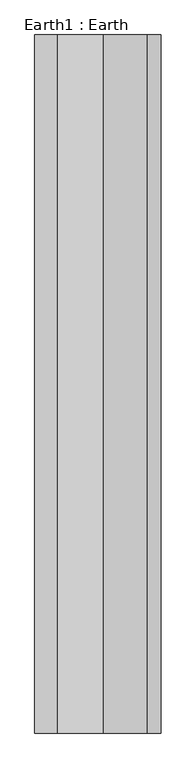
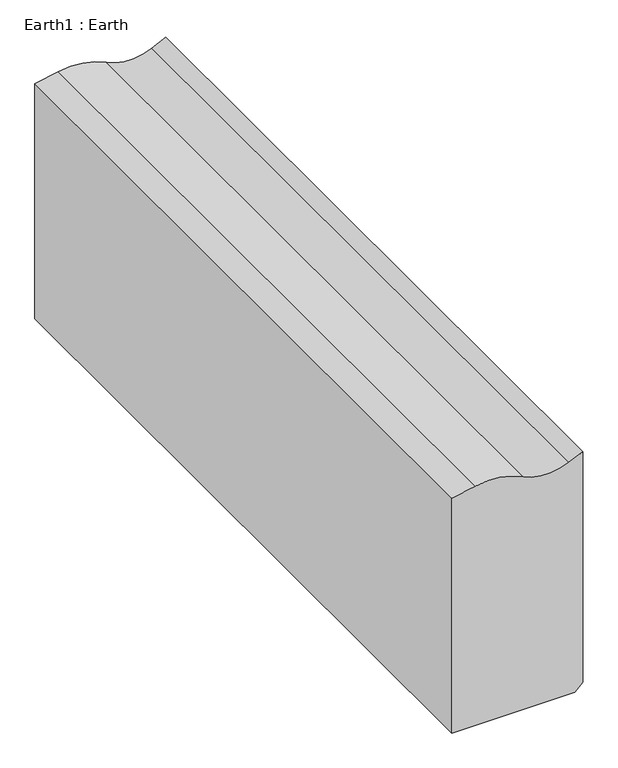
"""IFC4 building model written with IfcOpenShell, lengths in millimetres: proxy geometry, Earth1 : Earth."""

from ifc_helpers import new_model, si_unit, point, frame, frame_2d, origin, place, context, project, spatial, polyline, circle_curve, trimmed, segment, composite_curve, outline, extrude, source, transform, mapped, element, save


def earth1_earth_1ffde3c4(model_context):
    return source(origin(), model_context, "Body", "SweptSolid", [
        extrude(outline(composite_curve([segment(polyline([(32620.9902343, -10057.5706312), (32620.9902343, -9717.2148439), (32643.1028304, -9695.1022478), (33318.0501956, -9695.1022478), (33300.0908366, -9733.8927957)]), True, "CONTINUOUS"), segment(trimmed(circle_curve(frame_2d((33431.3167137, -9794.6481283)), 144.607888), [point((33300.0908366, -9733.8927957))], [point((33302.6181918, -9860.5884932))], True, "CARTESIAN"), True, "CONTINUOUS"), segment(trimmed(circle_curve(frame_2d((33120.1913863, -9954.0572443)), 204.9779178), [point((33302.6181918, -9860.5884932))], [point((33321.4784396, -9992.7802216))], False, "CARTESIAN"), True, "CONTINUOUS"), segment(polyline([(33321.4784396, -9992.7802216), (33309.014262, -10057.5706312), (32620.9902343, -10057.5706312)]), True, "CONTINUOUS")], self_intersect=False)), frame((0.0, 7982.1531721, 0.0), z_axis=(0.0, 1.0, 0.0), x_axis=(0.0, 0.0, 1.0)), (0.0, 0.0, 1.0), 2000.0),
    ])


if __name__ == "__main__":
    model = new_model("IFC4")
    model_context = context("Model", 3, world=origin())
    ifc_project = project(units=[si_unit("LENGTHUNIT", "METRE", prefix="MILLI")], contexts=[model_context])
    site = spatial("IfcSite", under=ifc_project)
    building = spatial("IfcBuilding", under=site)
    placement = place(None, origin())
    earth1_earth_shape = earth1_earth_1ffde3c4(model_context)
    element("IfcBuildingElementProxy", 1, Name="Earth1 : Earth", ObjectType="Earth1 : Earth", at=placement, inside=building, context=model_context, shape_type="MappedRepresentation", body=[
        mapped(earth1_earth_shape, transform((0.0, 0.0, 0.0), x_axis=(1.0, 0.0, 0.0), y_axis=(0.0, 1.0, 0.0), z_axis=(0.0, 0.0, 1.0))),
    ])
    save(model, "model.ifc")

# Revit data of these elements
# Type "Earth1 : Earth"
#   NameOverride = "Earth"
# Element 1 (IfcBuildingElementProxy, "Earth1 : Earth")
#   Materials on its faces: "GROUND SOIL"
# Materials
#   "GROUND SOIL": class "Unassigned", colour RGB 170 124 75, transparency 0, Cost = 0
